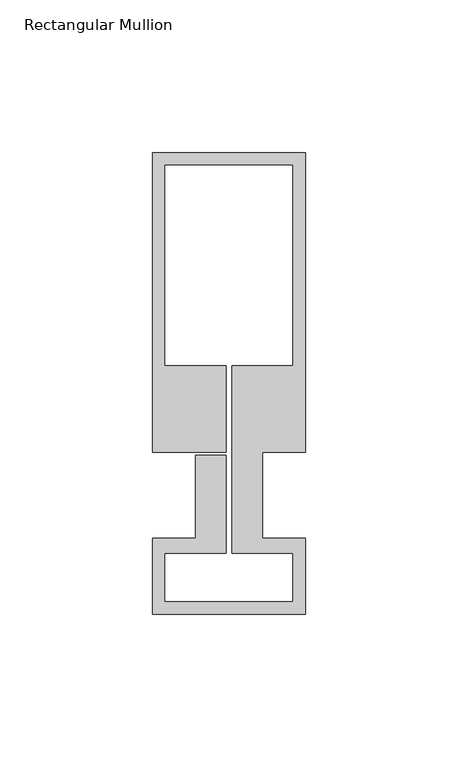
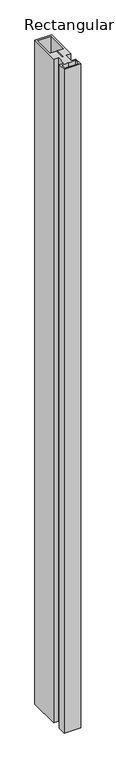
"""IFC4 building model written with IfcOpenShell, lengths in millimetres: member geometry, Rectangular Mullion : Schueco_FWS-50-HI_Mull_CovCap-20mm_Mull-85mm."""

from ifc_helpers import new_model, si_unit, frame, origin, place, context, project, spatial, polyline, outline, extrude, source, transform, mapped, element, save


def rectangular_mullion_cc323336(model_context):
    return source(origin(), model_context, "Body", "SweptSolid", [
        extrude(outline(polyline([(25.0, 126.0), (25.0, 28.0), (11.0, 28.0), (11.0, -0.1), (25.0, -0.1), (25.0, -25.0), (-25.0, -25.0), (-25.0, -0.1), (-11.0, -0.1), (-11.0, 27.0), (-1.0, 27.0), (-1.0, -5.0), (-21.0, -5.0), (-21.0, -21.0), (21.0, -21.0), (21.0, -5.0), (1.0, -5.0), (1.0, 56.3), (21.0, 56.3), (21.0, 122.0), (-21.0, 122.0), (-21.0, 56.3), (-1.0, 56.3), (-1.0, 28.0), (-25.0, 28.0), (-25.0, 126.0), (25.0, 126.0)])), frame((0.0, 0.0, -2100.0), z_axis=(0.0, 0.0, 1.0), x_axis=(1.0, 0.0, 0.0)), (0.0, 0.0, 1.0), 2100.0),
    ])


if __name__ == "__main__":
    model = new_model("IFC4")
    model_context = context("Model", 3, world=origin())
    ifc_project = project(units=[si_unit("LENGTHUNIT", "METRE", prefix="MILLI")], contexts=[model_context])
    site = spatial("IfcSite", under=ifc_project)
    building = spatial("IfcBuilding", under=site)
    placement = place(None, origin())
    rectangular_mullion_shape = rectangular_mullion_cc323336(model_context)
    element("IfcMember", 1, ObjectType="Rectangular Mullion : Schueco_FWS-50-HI_Mull_CovCap-20mm_Mull-85mm", at=placement, inside=building, context=model_context, shape_type="MappedRepresentation", body=[
        mapped(rectangular_mullion_shape, transform((0.0, 0.0, 0.0), x_axis=(1.0, 0.0, 0.0), y_axis=(0.0, 1.0, 0.0), z_axis=(0.0, 0.0, 1.0))),
    ])
    save(model, "model.ifc")

# Revit data of these elements
# Type "Rectangular Mullion : Schueco_FWS-50-HI_Mull_CovCap-20mm_Mull-85mm"
#   Model = "FWS 50.HI"
#   Manufacturer = "Schueco International KG"
#   Type Comments = "Mullion"
#   Schueco thermal insulation standard = "Highly thermally insulated"
#   Burglar resistance = "RC 3"
#   Thermal insulation = "to 0.90 W/(m²K)"
#   built-in parameter 1007322 = 0.495407 (stored number, unit not read)
#   built-in parameter 1007321 = 0.0360892 (stored number, unit not read)
#   built-in parameter 1007320 = 0.0360892 (stored number, unit not read)
# Element 1 (IfcMember, "Rectangular Mullion : Schueco_FWS-50-HI_Mull_CovCap-20mm_Mull-85mm")
#   Materials on its faces: "Alu"
# Materials
#   "Alu": class "Glas", colour RGB 140 140 140, transparency 0
